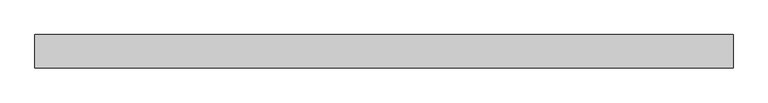
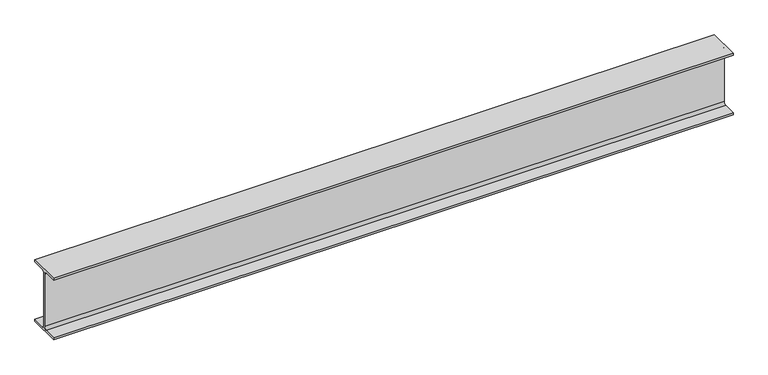
"""IFC4 building model written with IfcOpenShell, lengths in millimetres: beam geometry, 0912_Steel Framing_H-KSD3502 : H_SB_ASB_H-350x175x7x11."""

from ifc_helpers import new_model, si_unit, point, frame, frame_2d, origin, place, context, project, spatial, polyline, circle_curve, trimmed, segment, composite_curve, outline, extrude, source, transform, mapped, element, save


def beam_954b2bf2(model_context):
    return source(origin(), model_context, "Body", "SweptSolid", [
        extrude(outline(composite_curve([segment(polyline([(87.5, -164.0), (87.5, -175.0), (-87.5, -175.0), (-87.5, -164.0), (-17.5, -164.0)]), True, "CONTINUOUS"), segment(trimmed(circle_curve(frame_2d((-17.5, -150.0)), 14.0), [point((-17.5, -164.0))], [point((-3.5, -150.0))], True, "CARTESIAN"), True, "CONTINUOUS"), segment(polyline([(-3.5, -150.0), (-3.5, 150.0)]), True, "CONTINUOUS"), segment(trimmed(circle_curve(frame_2d((-17.5, 150.0)), 14.0), [point((-3.5, 150.0))], [point((-17.5, 164.0))], True, "CARTESIAN"), True, "CONTINUOUS"), segment(polyline([(-17.5, 164.0), (-87.5, 164.0), (-87.5, 175.0), (87.5, 175.0), (87.5, 164.0), (17.5, 164.0)]), True, "CONTINUOUS"), segment(trimmed(circle_curve(frame_2d((17.5, 150.0)), 14.0), [point((17.5, 164.0))], [point((3.5, 150.0))], True, "CARTESIAN"), True, "CONTINUOUS"), segment(polyline([(3.5, 150.0), (3.5, -150.0)]), True, "CONTINUOUS"), segment(trimmed(circle_curve(frame_2d((17.5, -150.0)), 14.0), [point((3.5, -150.0))], [point((17.5, -164.0))], True, "CARTESIAN"), True, "CONTINUOUS"), segment(polyline([(17.5, -164.0), (87.5, -164.0)]), True, "CONTINUOUS")], self_intersect=False)), frame((-1837.3, 0.0, 0.0), z_axis=(1.0, 0.0, 0.0), x_axis=(0.0, 1.0, 0.0)), (0.0, 0.0, 1.0), 3674.6),
    ])


if __name__ == "__main__":
    model = new_model("IFC4")
    model_context = context("Model", 3, world=origin())
    ifc_project = project(units=[si_unit("LENGTHUNIT", "METRE", prefix="MILLI")], contexts=[model_context])
    site = spatial("IfcSite", under=ifc_project)
    building = spatial("IfcBuilding", under=site)
    placement = place(None, origin())
    beam_shape = beam_954b2bf2(model_context)
    element("IfcBeam", 1, ObjectType="0912_Steel Framing_H-KSD3502 : H_SB_ASB_H-350x175x7x11", at=placement, inside=building, context=model_context, shape_type="MappedRepresentation", body=[
        mapped(beam_shape, transform((0.0, 0.0, 0.0), x_axis=(1.0, 0.0, 0.0), y_axis=(0.0, 1.0, 0.0), z_axis=(0.0, 0.0, 1.0))),
    ])
    save(model, "model.ifc")

# Revit data of these elements
# Type "0912_Steel Framing_H-KSD3502 : H_SB_ASB_H-350x175x7x11"
#   H_WM Code_1 = "S01AA002-00001 | Main Steel Structure Fabrication Work | Shelter/Building | Medium Steel - Standard (90KG/M>Weight≥30KG/M) | Material: (   )"
#   H_WM Code_2 = "S03AA028-00001 | Main Steel Structure Erection Work | Shelter/Building | Medium Steel (90KG/M>Weight≥30KG/M) | Material: (   )"
#   H_WM Code_3 = "S01AA010-00001 | Main Steel Structure Fabrication Work | Shelter/Building | Steel Painting/Coating | for Non-Fireproofed Steel Surface, Surface Preparation, Primer, Second & Final Coat | Material: (   )"
#   H_Q'ty Cal Type Tag = "SB-Q2"
#   Width = 17.5 cm
#   Web Thickness = 0.7 cm
#   Web Fillet = 1.4 cm
#   Warping Constant = 282000.0 cm⁶
#   W = 0
#   Torsional Moment of Inertia = 19.4042 cm⁴
#   Section Area = 63.14 cm²
#   Plastic Modulus weak axis = 174.0 cm³
#   Plastic Modulus strong axis = 868.0 cm³
#   Perimeter = 1.36 m²/m
#   Nominal Weight = 49.60 kgf/m
#   Moment of Inertia weak axis = 984.00 cm⁴
#   Moment of Inertia strong axis = 13600.00 cm⁴
#   Height = 35.0 cm
#   Flange Thickness = 1.1 cm
#   Elastic Modulus weak axis = 112.0 cm³
#   Elastic Modulus strong axis = 775.0 cm³
#   Centroid Vertical = 17.5 cm
#   Centroid Horizontal = 8.75 cm
#   Ix = 136000000
#   Length [instance default] = 1.5240 m
#   Zx = 868000
#   b = 0.1750 m
#   h = 0.3500 m
#   r = 0.0140 m
#   s = 0.0070 m
#   t = 0.0110 m
#   A = 0.006314 m²
#   Structural Material [instance default] = Steel, 45-345
#   Assembly Code = ""
# Element 1 (IfcBeam, "0912_Steel Framing_H-KSD3502 : H_SB_ASB_H-350x175x7x11")
#   Structural Material = none
# Materials
#   "Steel, 45-345": class "Metal", colour RGB 189 187 185, transparency 0, Description = "Steel 345 MPa", Cost = 0
